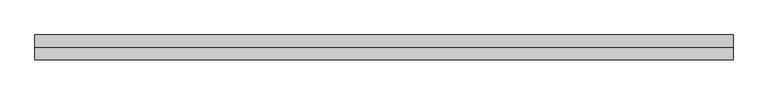
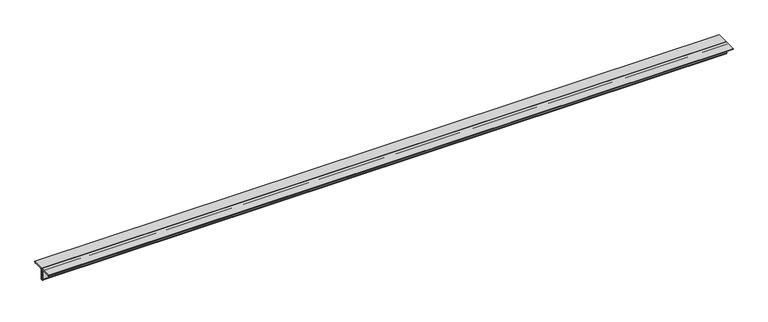
"""IFC4 building model written with IfcOpenShell, lengths in millimetres: member geometry, Steel Framing_2Ls_KS : H_SB_AR_S02_2Ls-100x100x10_VBR1."""

from ifc_helpers import new_model, si_unit, point, frame, frame_2d, origin, place, context, project, spatial, polyline, circle_curve, trimmed, segment, composite_curve, outline, extrude, source, transform, mapped, element, save


def member_685a7afe(model_context):
    return source(origin(), model_context, "Body", "SweptSolid", [
        extrude(outline(composite_curve([segment(polyline([(0.0, 28.2), (100.0, 28.2)]), True, "CONTINUOUS"), segment(trimmed(circle_curve(frame_2d((90.0, 28.2)), 10.0), [point((100.0, 28.2))], [point((90.0, 18.2))], False, "CARTESIAN"), True, "CONTINUOUS"), segment(polyline([(90.0, 18.2), (20.0, 18.2)]), True, "CONTINUOUS"), segment(trimmed(circle_curve(frame_2d((20.0, 8.2)), 10.0), [point((20.0, 18.2))], [point((10.0, 8.2))], True, "CARTESIAN"), True, "CONTINUOUS"), segment(polyline([(10.0, 8.2), (10.0, -61.8)]), True, "CONTINUOUS"), segment(trimmed(circle_curve(frame_2d((0.0, -61.8)), 10.0), [point((10.0, -61.8))], [point((0.0, -71.8))], False, "CARTESIAN"), True, "CONTINUOUS"), segment(polyline([(0.0, -71.8), (0.0, 28.2)]), True, "CONTINUOUS")], self_intersect=False)), frame((-2765.2972366, 0.0, 0.0), z_axis=(1.0, 0.0, 0.0), x_axis=(0.0, 1.0, 0.0)), (0.0, 0.0, 1.0), 5642.6869734),
        extrude(outline(composite_curve([segment(polyline([(0.0, 28.2), (0.0, -71.8)]), True, "CONTINUOUS"), segment(trimmed(circle_curve(frame_2d((0.0, -61.8)), 10.0), [point((0.0, -71.8))], [point((-10.0, -61.8))], False, "CARTESIAN"), True, "CONTINUOUS"), segment(polyline([(-10.0, -61.8), (-10.0, 8.2)]), True, "CONTINUOUS"), segment(trimmed(circle_curve(frame_2d((-20.0, 8.2)), 10.0), [point((-10.0, 8.2))], [point((-20.0, 18.2))], True, "CARTESIAN"), True, "CONTINUOUS"), segment(polyline([(-20.0, 18.2), (-90.0, 18.2)]), True, "CONTINUOUS"), segment(trimmed(circle_curve(frame_2d((-90.0, 28.2)), 10.0), [point((-90.0, 18.2))], [point((-100.0, 28.2))], False, "CARTESIAN"), True, "CONTINUOUS"), segment(polyline([(-100.0, 28.2), (0.0, 28.2)]), True, "CONTINUOUS")], self_intersect=False)), frame((-2765.2972366, 0.0, 0.0), z_axis=(1.0, 0.0, 0.0), x_axis=(0.0, 1.0, 0.0)), (0.0, 0.0, 1.0), 5642.6869734),
    ])


if __name__ == "__main__":
    model = new_model("IFC4")
    model_context = context("Model", 3, world=origin())
    ifc_project = project(units=[si_unit("LENGTHUNIT", "METRE", prefix="MILLI")], contexts=[model_context])
    site = spatial("IfcSite", under=ifc_project)
    building = spatial("IfcBuilding", under=site)
    placement = place(None, origin())
    member_shape = member_685a7afe(model_context)
    element("IfcMember", 1, ObjectType="Steel Framing_2Ls_KS : H_SB_AR_S02_2Ls-100x100x10_VBR1", at=placement, inside=building, context=model_context, shape_type="MappedRepresentation", body=[
        mapped(member_shape, transform((0.0, 0.0, 0.0), x_axis=(1.0, 0.0, 0.0), y_axis=(0.0, 1.0, 0.0), z_axis=(0.0, 0.0, 1.0))),
    ])
    save(model, "model.ifc")

# Revit data of these elements
# Type "Steel Framing_2Ls_KS : H_SB_AR_S02_2Ls-100x100x10_VBR1"
#   Type Comments = "MAIN"
#   Type Mark = "VBR1"
#   H_SectionID = "2Ls-100x100x10"
#   Assembly Code = "B10"
#   Legs = "LLBB"
#   H_Ratio for Additional Steel Plate = 0.2
#   W = 0
#   Perimeter = 0.80 m²/m
#   Nominal Weight = 29.80 kgf/m
#   Length [instance default] = 1524 mm
#   Space = 0 mm
#   b = 100 mm
#   d = 100 mm
#   t = 10 mm
#   y = 28.2 mm
#   A = 0.0038 m²
#   Structural Material [instance default] = Steel, 45-345
# Element 1 (IfcMember, "Steel Framing_2Ls_KS : H_SB_AR_S02_2Ls-100x100x10_VBR1")
#   Materials on its faces: "Steel, 45-345"
# Materials
#   "Steel, 45-345": class "Metal", colour RGB 189 187 185, transparency 0, Description = "Steel 345 MPa", Cost = 0
